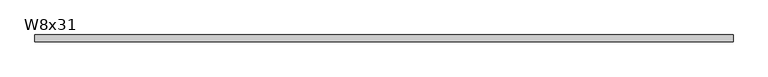
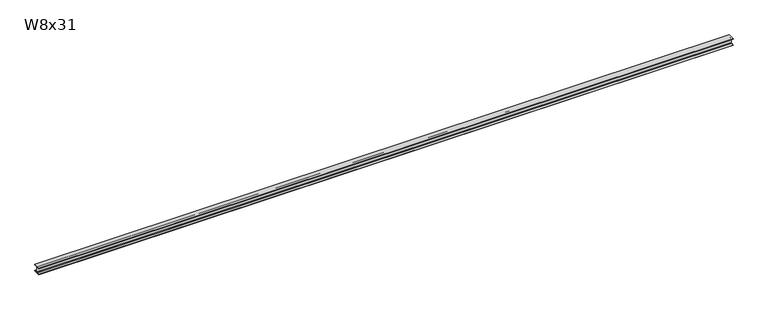
"""IFC4 building model written with IfcOpenShell, lengths in millimetres: beam geometry, RME W-Wide Flange : W8x31."""

from ifc_helpers import new_model, si_unit, point, frame, frame_2d, origin, place, context, project, spatial, polyline, circle_curve, trimmed, segment, composite_curve, outline, extrude, source, transform, mapped, element, save


def w8x31_b47741b7(model_context):
    return source(origin(), model_context, "Body", "SweptSolid", [
        extrude(outline(composite_curve([segment(polyline([(101.6, -90.551), (101.6, -101.6), (-101.6, -101.6), (-101.6, -90.551), (-21.1455, -90.551)]), True, "CONTINUOUS"), segment(trimmed(circle_curve(frame_2d((-21.1455, -73.025)), 17.526), [point((-21.1455, -90.551))], [point((-3.6195, -73.025))], True, "CARTESIAN"), True, "CONTINUOUS"), segment(polyline([(-3.6195, -73.025), (-3.6195, 73.025)]), True, "CONTINUOUS"), segment(trimmed(circle_curve(frame_2d((-21.1455, 73.025)), 17.526), [point((-3.6195, 73.025))], [point((-21.1455, 90.551))], True, "CARTESIAN"), True, "CONTINUOUS"), segment(polyline([(-21.1455, 90.551), (-101.6, 90.551), (-101.6, 101.6), (101.6, 101.6), (101.6, 90.551), (21.1455, 90.551)]), True, "CONTINUOUS"), segment(trimmed(circle_curve(frame_2d((21.1455, 73.025)), 17.526), [point((21.1455, 90.551))], [point((3.6195, 73.025))], True, "CARTESIAN"), True, "CONTINUOUS"), segment(polyline([(3.6195, 73.025), (3.6195, -73.025)]), True, "CONTINUOUS"), segment(trimmed(circle_curve(frame_2d((21.1455, -73.025)), 17.526), [point((3.6195, -73.025))], [point((21.1455, -90.551))], True, "CARTESIAN"), True, "CONTINUOUS"), segment(polyline([(21.1455, -90.551), (101.6, -90.551)]), True, "CONTINUOUS")], self_intersect=False)), frame((-10228.5871156, 0.0, 0.0), z_axis=(1.0, 0.0, 0.0), x_axis=(0.0, 1.0, 0.0)), (0.0, 0.0, 1.0), 20457.1742311),
    ])


if __name__ == "__main__":
    model = new_model("IFC4")
    model_context = context("Model", 3, world=origin())
    ifc_project = project(units=[si_unit("LENGTHUNIT", "METRE", prefix="MILLI")], contexts=[model_context])
    site = spatial("IfcSite", under=ifc_project)
    building = spatial("IfcBuilding", under=site)
    placement = place(None, origin())
    w8x31_shape = w8x31_b47741b7(model_context)
    element("IfcBeam", 1, ObjectType="RME W-Wide Flange : W8x31", at=placement, inside=building, context=model_context, shape_type="MappedRepresentation", body=[
        mapped(w8x31_shape, transform((0.0, 0.0, 0.0), x_axis=(1.0, 0.0, 0.0), y_axis=(0.0, 1.0, 0.0), z_axis=(0.0, 0.0, 1.0))),
    ])
    save(model, "model.ifc")

# Revit data of these elements
# Type "RME W-Wide Flange : W8x31"
#   WELD P [instance default] = ""
#   WELD LE [instance default] = ""
#   WELD D [instance default] = ""
#   TOP SECTION SIZE [instance default] = ""
#   TOP SECTION LENGTH [instance default] = ""
#   REMARKS [instance default] = ""
#   REINF TYPE [instance default] = ""
#   Nominal Size = "W24"
#   End Bearing Capacity [instance default] = ""
#   BOT SECTION SIZE [instance default] = ""
#   BOT SECTION LENGTH [instance default] = ""
#   Assembly Code = "B10"
#   W = 31
#   Start Extension Calculation [instance default] = 10' - 0"
#   Start Extension [instance default] = -0' - 0 1/2"
#   End Extension Calculation [instance default] = 10' - 0"
#   End Extension [instance default] = -0' - 0 1/2"
#   Length [instance default] = 5' - 0"
#   bf = 0' - 8"
#   d = 0' - 8"
#   k = 0' - 1 1/8"
#   k2 = 0' - 0.69"
#   tf = 0' - 0.435"
#   tw = 0' - 0.285"
#   A = 0.0633333 SF
#   Structural Material [instance default] = Metal - Steel - ASTM A992
# Element 1 (IfcBeam, "RME W-Wide Flange : W8x31")
#   Length = 67' - 1.40056"
#   Materials on its faces: "Metal - Steel - ASTM A992"
# Materials
#   "Metal - Steel - ASTM A992": class "Metal", colour RGB 255 128 0, transparency 0
